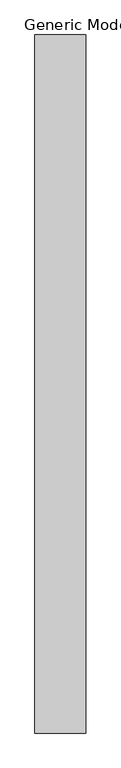
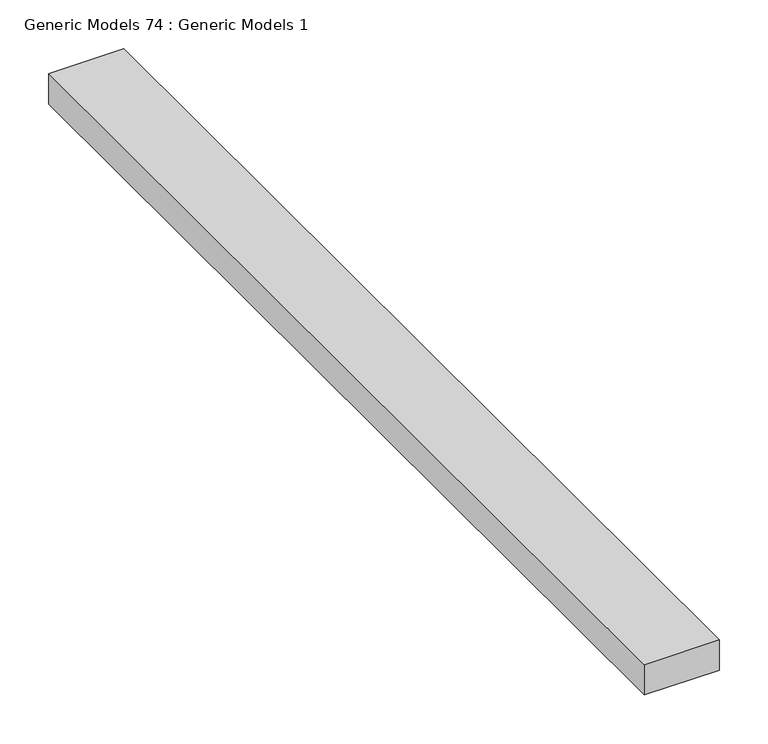
"""IFC4 building model written with IfcOpenShell, lengths in millimetres: proxy geometry, Generic Models 74 : Generic Models 1."""

from ifc_helpers import new_model, si_unit, frame, origin, place, context, project, spatial, polyline, outline, extrude, source, transform, mapped, element, save


def generic_models_74_generic_models_1_1398e35e(model_context):
    return source(origin(), model_context, "Body", "SweptSolid", [
        extrude(outline(polyline([(48561.625, 0.0), (48472.725, 0.0), (48472.725, 1219.2), (48561.625, 1219.2), (48561.625, 0.0)])), frame((0.0, 0.0, 2447.200412), z_axis=(0.0, 0.0, 1.0), x_axis=(1.0, 0.0, 0.0)), (0.0, 0.0, 1.0), 38.1),
    ])


if __name__ == "__main__":
    model = new_model("IFC4")
    model_context = context("Model", 3, world=origin())
    ifc_project = project(units=[si_unit("LENGTHUNIT", "METRE", prefix="MILLI")], contexts=[model_context])
    site = spatial("IfcSite", under=ifc_project)
    building = spatial("IfcBuilding", under=site)
    placement = place(None, origin())
    generic_models_74_generic_models_1_shape = generic_models_74_generic_models_1_1398e35e(model_context)
    element("IfcBuildingElementProxy", 1, Name="Generic Models 74 : Generic Models 1", ObjectType="Generic Models 74 : Generic Models 1", at=placement, inside=building, context=model_context, shape_type="MappedRepresentation", body=[
        mapped(generic_models_74_generic_models_1_shape, transform((0.0, 0.0, 0.0), x_axis=(1.0, 0.0, 0.0), y_axis=(0.0, 1.0, 0.0), z_axis=(0.0, 0.0, 1.0))),
    ])
    save(model, "model.ifc")

# Revit data of these elements
# Element 1 (IfcBuildingElementProxy, "Generic Models 74 : Generic Models 1")
#   Materials on its faces: "2X4 WOOD STUDS"
# Materials
#   "2X4 WOOD STUDS": class "Wood", colour RGB 144 113 62, transparency 0, Description = "Pinus Echinata", Cost = 0
